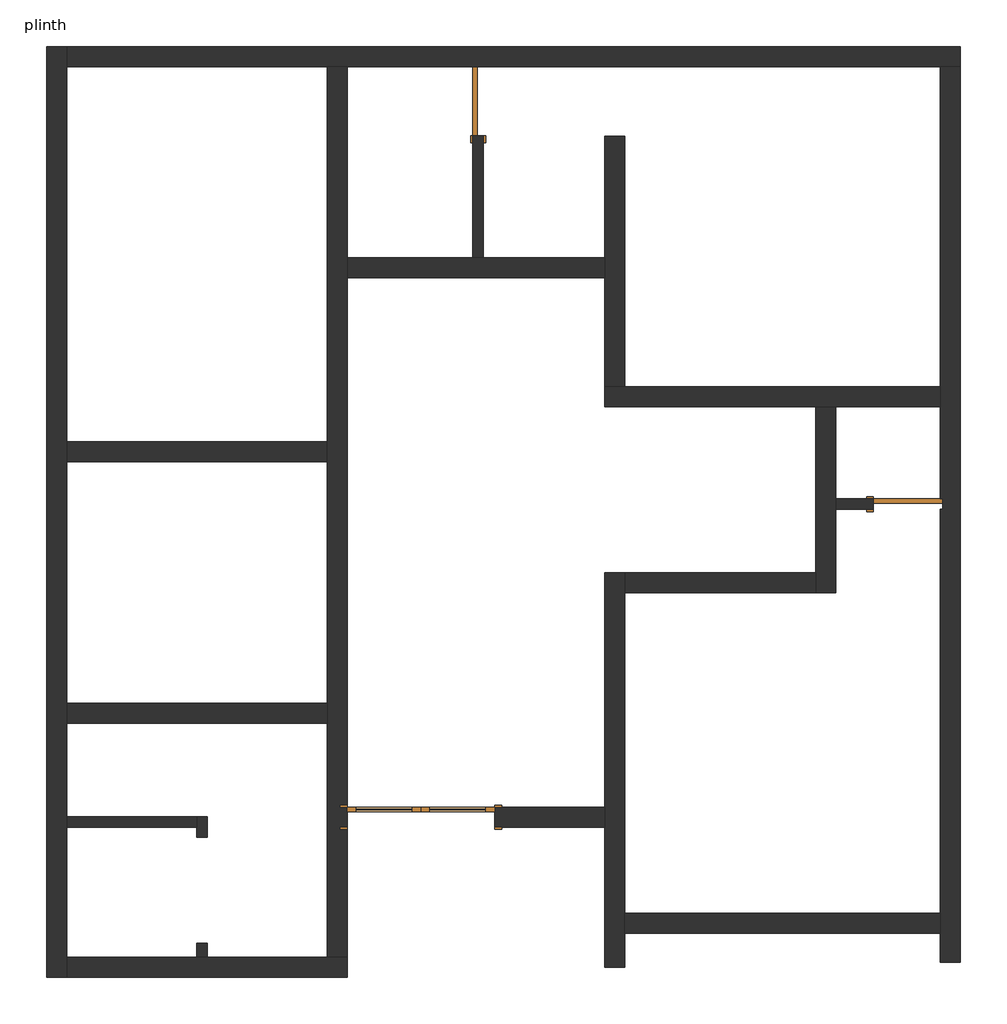
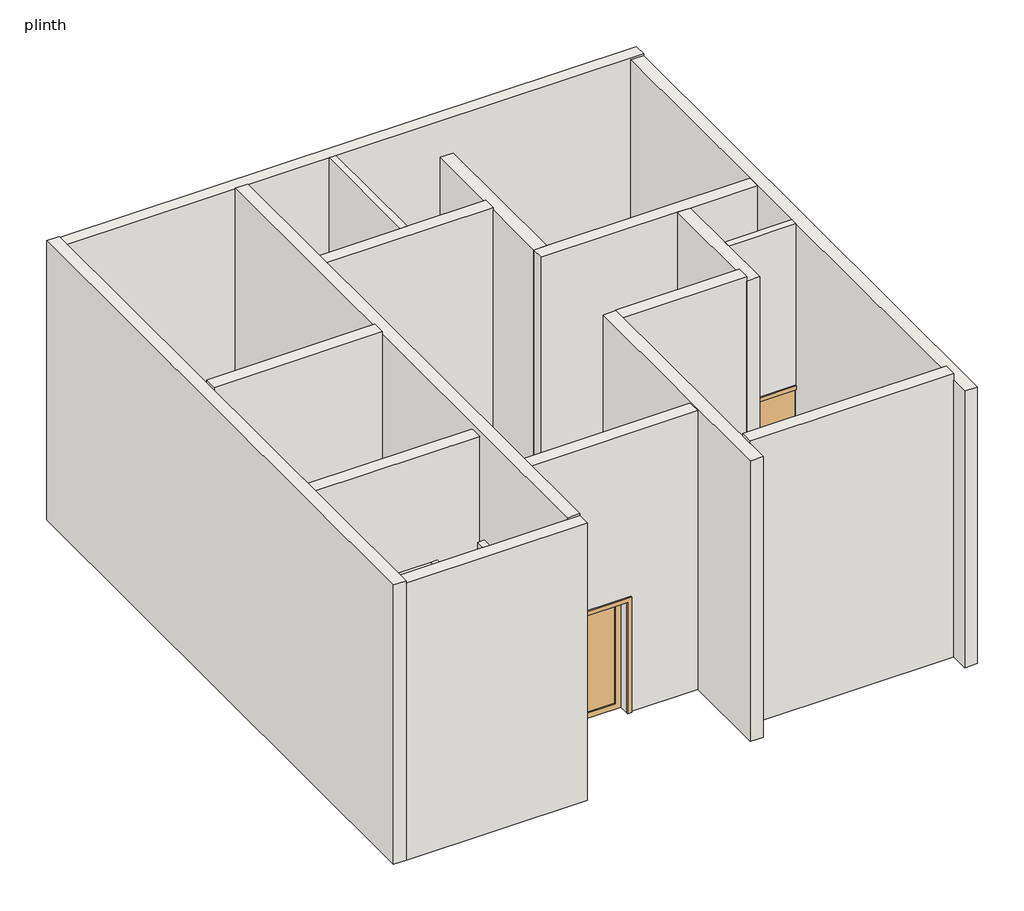
# One storey: 20 walls, 3 doors.
"""IFC4 building model written with IfcOpenShell, lengths in millimetres."""

import ifcopenshell
import ifcopenshell.guid

model = None  # the IFC model being written
_history = None  # IfcOwnerHistory: only IFC2X3 demands one
_inside = {}  # id of a spatial element -> (the spatial element, [elements in it])
_under = {}  # id of a project, library or spatial element -> (it, [spatial elements below it])
_declared = {}  # id of a project -> (the project, [libraries it declares])
_typed = {}  # id of a type object -> (the type object, [elements of that type])
_made_of = {}  # id of a material, layer set ... -> (it, [elements and type objects made of it])


def new_model(schema):
    """Start an empty IFC model of exactly this schema.

    Asked for "IFC4X3", IfcOpenShell would pick the latest addendum, in which some entities
    have other attributes; the version numbers below select the first issue.
    IFC2X3 requires an IfcOwnerHistory on every rooted entity: one is made here for all.
    """
    global model, _history
    if schema == "IFC4X3":
        model = ifcopenshell.file(schema_version=(4, 3, 0, 0))
    else:
        model = ifcopenshell.file(schema=schema)
    _inside.clear()
    _under.clear()
    _declared.clear()
    _typed.clear()
    _made_of.clear()
    _history = None
    if model.schema == "IFC2X3":
        org = make("IfcOrganization", Name="unknown")
        user = make(
            "IfcPersonAndOrganization",
            ThePerson=make("IfcPerson", FamilyName="unknown"),
            TheOrganization=org,
        )
        app = make(
            "IfcApplication",
            ApplicationDeveloper=org,
            Version="unknown",
            ApplicationFullName="unknown",
            ApplicationIdentifier="unknown",
        )
        _history = make(
            "IfcOwnerHistory",
            OwningUser=user,
            OwningApplication=app,
            ChangeAction="ADDED",
            CreationDate=0,
        )
    return model


def make(cls, **values):
    """One entity of the class cls with the attributes given. An attribute that is None is left unset."""
    return model.create_entity(
        cls, **{name: value for name, value in values.items() if value is not None}
    )


def rooted(cls, **values):
    """An entity with a GlobalId (a new one), such as an element, a storey or a relation."""
    return make(cls, GlobalId=ifcopenshell.guid.new(), OwnerHistory=_history, **values)


def si_unit(unit_type, name, prefix=None):
    """IfcSIUnit, for example si_unit("LENGTHUNIT", "METRE", prefix="MILLI")."""
    return make("IfcSIUnit", UnitType=unit_type, Prefix=prefix, Name=name)


def assignment(units):
    """IfcUnitAssignment: the units of a project."""
    return None if units is None else make("IfcUnitAssignment", Units=units)


def point(xyz):
    """IfcCartesianPoint."""
    return None if xyz is None else make("IfcCartesianPoint", Coordinates=xyz)


def direction(xyz):
    """IfcDirection."""
    return None if xyz is None else make("IfcDirection", DirectionRatios=xyz)


def frame(location, z_axis=None, x_axis=None):
    """IfcAxis2Placement3D, a coordinate frame: its origin and axes. An axis left out is left unset."""
    return make(
        "IfcAxis2Placement3D",
        Location=point(location),
        Axis=direction(z_axis),
        RefDirection=direction(x_axis),
    )


def origin():
    """The frame at (0, 0, 0) with its axes left unset."""
    return frame((0.0, 0.0, 0.0))


def origin_with_axes():
    """The frame at (0, 0, 0) with the z axis (0, 0, 1) and the x axis (1, 0, 0) written out."""
    return frame((0.0, 0.0, 0.0), z_axis=(0.0, 0.0, 1.0), x_axis=(1.0, 0.0, 0.0))


def place(relative_to, where):
    """IfcLocalPlacement: puts the frame where relative to a parent placement (None: the world)."""
    return make(
        "IfcLocalPlacement", PlacementRelTo=relative_to, RelativePlacement=where
    )


def context(
    kind, dimensions, precision=None, world=None, true_north=None, identifier=None
):
    """IfcGeometricRepresentationContext, for example the 3D "Model" context."""
    return make(
        "IfcGeometricRepresentationContext",
        ContextIdentifier=identifier,
        ContextType=kind,
        CoordinateSpaceDimension=dimensions,
        Precision=precision,
        WorldCoordinateSystem=world,
        TrueNorth=true_north,
    )


def project(units=None, contexts=None):
    """IfcProject with its units and contexts."""
    return rooted(
        "IfcProject",
        Name="project",
        RepresentationContexts=contexts,
        UnitsInContext=assignment(units),
    )


def spatial(cls, under=None, at=None, **own):
    """A site, building, storey or space (cls), placed at a placement, below another one or the project."""
    s = rooted(cls, ObjectPlacement=at, **own)
    if under is not None:
        _under.setdefault(under.id(), (under, []))[1].append(s)
    return s


def polyline(points):
    """IfcPolyline through the points."""
    return make("IfcPolyline", Points=[point(p) for p in points])


def outline(outer, holes=None, kind="AREA"):
    """IfcArbitraryClosedProfileDef: a profile drawn as a closed curve; with holes, ...WithVoids."""
    if holes is None:
        return make("IfcArbitraryClosedProfileDef", ProfileType=kind, OuterCurve=outer)
    return make(
        "IfcArbitraryProfileDefWithVoids",
        ProfileType=kind,
        OuterCurve=outer,
        InnerCurves=holes,
    )


def extrude(swept, where, along, depth):
    """IfcExtrudedAreaSolid: the profile swept, set in the frame where, extruded along a direction by depth."""
    return make(
        "IfcExtrudedAreaSolid",
        SweptArea=swept,
        Position=where,
        ExtrudedDirection=direction(along),
        Depth=depth,
    )


def faces_of(points, faces, orient=None, outer=None):
    """IfcFace entities. A face is a list of loops; a loop is a list of indices into points, from 0.

    orient and outer hold one flag for each loop. By default every Orientation is true, the
    first loop of a face is its IfcFaceOuterBound and the others are IfcFaceBound.
    """
    made = []
    for i, loops in enumerate(faces):
        bounds = []
        for j, loop in enumerate(loops):
            is_outer = j == 0 if outer is None else outer[i][j]
            bounds.append(
                make(
                    "IfcFaceOuterBound" if is_outer else "IfcFaceBound",
                    Bound=make("IfcPolyLoop", Polygon=[points[k] for k in loop]),
                    Orientation=True if orient is None else orient[i][j],
                )
            )
        made.append(make("IfcFace", Bounds=bounds))
    return made


def faceted_brep(points, faces, orient=None, outer=None, voids=None):
    """IfcFacetedBrep: a solid bounded by flat faces; with voids (closed shells), ...WithVoids."""
    shared = [point(p) for p in points]
    hull = make("IfcClosedShell", CfsFaces=faces_of(shared, faces, orient, outer))
    if voids is None:
        return make("IfcFacetedBrep", Outer=hull)
    return make(
        "IfcFacetedBrepWithVoids",
        Outer=hull,
        Voids=[
            make(cls, CfsFaces=faces_of(shared, fs, o, b)) for cls, fs, o, b in voids
        ],
    )


def shape(context_of_items, identifier, shape_type, items):
    """IfcShapeRepresentation: the items that make up one representation, for example the "Body"."""
    return make(
        "IfcShapeRepresentation",
        ContextOfItems=context_of_items,
        RepresentationIdentifier=identifier,
        RepresentationType=shape_type,
        Items=items,
    )


def source(mapping_origin, context_of_items, identifier, shape_type, items):
    """IfcRepresentationMap: a shape defined once, which mapped items show again and again."""
    return make(
        "IfcRepresentationMap",
        MappingOrigin=mapping_origin,
        MappedRepresentation=shape(context_of_items, identifier, shape_type, items),
    )


def transform(
    local_origin,
    x_axis=None,
    y_axis=None,
    z_axis=None,
    scale=None,
    scale2=None,
    scale3=None,
    uniform=True,
):
    """IfcCartesianTransformationOperator3D, or its non-uniform kind. x_axis, y_axis, z_axis: its Axis1, 2, 3."""
    if uniform:
        return make(
            "IfcCartesianTransformationOperator3D",
            Axis1=direction(x_axis),
            Axis2=direction(y_axis),
            LocalOrigin=point(local_origin),
            Scale=scale,
            Axis3=direction(z_axis),
        )
    return make(
        "IfcCartesianTransformationOperator3DnonUniform",
        Axis1=direction(x_axis),
        Axis2=direction(y_axis),
        LocalOrigin=point(local_origin),
        Scale=scale,
        Axis3=direction(z_axis),
        Scale2=scale2,
        Scale3=scale3,
    )


def mapped(mapping_source, mapping_target):
    """IfcMappedItem: shows the shape of a source again, moved by a transform."""
    return make(
        "IfcMappedItem", MappingSource=mapping_source, MappingTarget=mapping_target
    )


def made_of(thing, what):
    """Note that an element or type object is made of a material, layer set ...; save() writes the relation."""
    if what is not None:
        _made_of.setdefault(what.id(), (what, []))[1].append(thing)
    return thing


def element(
    cls,
    number,
    at=None,
    inside=None,
    cuts=None,
    type_object=None,
    material=None,
    context=None,
    identifier="Body",
    shape_type=None,
    held_by="IfcProductDefinitionShape",
    body=None,
    shapes=None,
    **own,
):
    """One element of the class cls, such as IfcWall. Its Tag is "e" and its number.

    at: its placement. inside: the storey or other place that contains it. cuts: it is an
    opening in that element (IfcRelVoidsElement). A single representation is given by context,
    identifier, shape_type and body (its items); several are given by shapes. held_by: the class
    of the entity that holds the representations. save() writes the other relations.
    """
    e = rooted(cls, Tag="e%d" % number, ObjectPlacement=at, **own)
    if body is not None:
        shapes = [shape(context, identifier, shape_type, body)]
    if shapes is not None:
        e.Representation = make(held_by, Representations=shapes)
    if inside is not None:
        _inside.setdefault(inside.id(), (inside, []))[1].append(e)
    if cuts is not None:
        rooted(
            "IfcRelVoidsElement", RelatingBuildingElement=cuts, RelatedOpeningElement=e
        )
    if type_object is not None:
        _typed.setdefault(type_object.id(), (type_object, []))[1].append(e)
    return made_of(e, material)


def aggregate(whole, parts):
    """IfcRelAggregates: a whole, such as a stair, and the parts it consists of."""
    return rooted("IfcRelAggregates", RelatingObject=whole, RelatedObjects=parts)


def save(model, path):
    """Write the relations noted so far, then the file.

    IfcRelAggregates (storeys below a building ...), IfcRelContainedInSpatialStructure (elements
    in a storey), IfcRelDefinesByType, IfcRelAssociatesMaterial and IfcRelDeclares: one each for
    every whole, place, type object, material and project.
    """
    for whole, parts in _under.values():
        aggregate(whole, parts)
    for where, things in _inside.values():
        rooted(
            "IfcRelContainedInSpatialStructure",
            RelatedElements=things,
            RelatingStructure=where,
        )
    for kind, things in _typed.values():
        rooted("IfcRelDefinesByType", RelatedObjects=things, RelatingType=kind)
    for what, things in _made_of.values():
        rooted("IfcRelAssociatesMaterial", RelatedObjects=things, RelatingMaterial=what)
    for by, libraries in _declared.values():
        rooted("IfcRelDeclares", RelatingContext=by, RelatedDefinitions=libraries)
    model.write(path)


def m_door_double_glass_1700_x_2100mm_d150df18(model_context):
    return source(origin(), model_context, "Body", "SweptSolid", [
        extrude(outline(polyline([(2100.0, -850.0), (0.0, -850.0), (0.0, 0.0), (2100.0, 0.0), (2100.0, -850.0)]), holes=[polyline([(2000.0, -750.0), (2000.0, -100.0), (100.0, -100.0), (100.0, -750.0), (2000.0, -750.0)])]), frame((0.0, 67.38125, 0.0), z_axis=(0.0, 1.0, 0.0), x_axis=(0.0, 0.0, 1.0)), (0.0, 0.0, 1.0), 50.0),
        extrude(outline(polyline([(2100.0, 850.0), (2100.0, 0.0), (0.0, 0.0), (0.0, 850.0), (2100.0, 850.0)]), holes=[polyline([(2000.0, 750.0), (100.0, 750.0), (100.0, 100.0), (2000.0, 100.0), (2000.0, 750.0)])]), frame((0.0, 67.38125, 0.0), z_axis=(0.0, 1.0, 0.0), x_axis=(0.0, 0.0, 1.0)), (0.0, 0.0, 1.0), 50.0),
        extrude(outline(polyline([(100.0, 95.55625), (750.0, 95.55625), (750.0, 89.20625), (100.0, 89.20625), (100.0, 95.55625)])), frame((0.0, 0.0, 100.0), z_axis=(0.0, 0.0, 1.0), x_axis=(1.0, 0.0, 0.0)), (0.0, 0.0, 1.0), 1900.0),
        extrude(outline(polyline([(-750.0, 95.55625), (-100.0, 95.55625), (-100.0, 89.20625), (-750.0, 89.20625), (-750.0, 95.55625)])), frame((0.0, 0.0, 100.0), z_axis=(0.0, 0.0, 1.0), x_axis=(1.0, 0.0, 0.0)), (0.0, 0.0, 1.0), 1900.0),
        extrude(outline(polyline([(0.0, 930.0), (2180.0, 930.0), (2180.0, -930.0), (0.0, -930.0), (0.0, -850.0), (2100.0, -850.0), (2100.0, 850.0), (0.0, 850.0), (0.0, 930.0)])), frame((0.0, 117.38125, 0.0), z_axis=(0.0, 1.0, 0.0), x_axis=(0.0, 0.0, 1.0)), (0.0, 0.0, 1.0), 25.0),
        extrude(outline(polyline([(0.0, 930.0), (2180.0, 930.0), (2180.0, -930.0), (0.0, -930.0), (0.0, -850.0), (2100.0, -850.0), (2100.0, 850.0), (0.0, 850.0), (0.0, 930.0)])), frame((0.0, -137.61875, 0.0), z_axis=(0.0, 1.0, 0.0), x_axis=(0.0, 0.0, 1.0)), (0.0, 0.0, 1.0), 25.0),
    ])


def m_door_single_panel_800_x_2100mm_7e59a417(model_context):
    return source(origin(), model_context, "Body", "SweptSolid", [
        extrude(outline(polyline([(400.0, 10.0), (-400.0, 10.0), (-400.0, 60.0), (400.0, 60.0), (400.0, 10.0)])), origin_with_axes(), (0.0, 0.0, 1.0), 2100.0),
        extrude(outline(polyline([(2176.2, -476.2), (0.0, -476.2), (0.0, -400.0), (2100.0, -400.0), (2100.0, 400.0), (0.0, 400.0), (0.0, 476.2), (2176.2, 476.2), (2176.2, -476.2)])), frame((0.0, 60.0, 0.0), z_axis=(0.0, 1.0, 0.0), x_axis=(0.0, 0.0, 1.0)), (0.0, 0.0, 1.0), 25.0),
        extrude(outline(polyline([(2176.2, 476.2), (2176.2, -476.2), (0.0, -476.2), (0.0, -400.0), (2100.0, -400.0), (2100.0, 400.0), (0.0, 400.0), (0.0, 476.2), (2176.2, 476.2)])), frame((0.0, -85.0, 0.0), z_axis=(0.0, 1.0, 0.0), x_axis=(0.0, 0.0, 1.0)), (0.0, 0.0, 1.0), 25.0),
    ])


model = new_model("IFC4")

# Units and contexts
model_context = context("Model", 3, world=origin())
ifc_project = project(units=[si_unit("LENGTHUNIT", "METRE", prefix="MILLI")], contexts=[model_context])

# Site, building, storey
site = spatial("IfcSite", under=ifc_project)
building = spatial("IfcBuilding", under=site)
storey = spatial("IfcBuildingStorey", under=building, Name="plinth", Elevation=450.0)

# Doors
placement = place(None, origin())
m_door_double_glass_1700_x_2100mm_shape = m_door_double_glass_1700_x_2100mm_d150df18(model_context)
element("IfcDoor", 1, ObjectType="M_Door-Double-Glass : 1700 x 2100mm", at=placement, inside=storey, context=model_context, shape_type="MappedRepresentation", body=[
    mapped(m_door_double_glass_1700_x_2100mm_shape, transform((-60244.5979307, 16200.8803218, 450.0), x_axis=(1.0, 0.0, 0.0), y_axis=(0.0, 1.0, 0.0), z_axis=(0.0, 0.0, 1.0))),
])
m_door_single_panel_800_x_2100mm_shape = m_door_single_panel_800_x_2100mm_7e59a417(model_context)
element("IfcDoor", 2, ObjectType="M_Door-Single-Panel : 800 x 2100mm", at=placement, inside=storey, context=model_context, shape_type="MappedRepresentation", body=[
    mapped(m_door_single_panel_800_x_2100mm_shape, transform((-54634.742358, 19808.2615718, 450.0), x_axis=(1.0, 0.0, 0.0), y_axis=(0.0, 1.0, 0.0), z_axis=(0.0, 0.0, 1.0))),
])
element("IfcDoor", 3, ObjectType="M_Door-Single-Panel : 800 x 2100mm", at=placement, inside=storey, context=model_context, shape_type="MappedRepresentation", body=[
    mapped(m_door_single_panel_800_x_2100mm_shape, transform((-59584.5979307, 24448.2615718, 450.0), x_axis=(0.0, 1.0, 0.0), y_axis=(-1.0, 0.0, 0.0), z_axis=(0.0, 0.0, 1.0))),
])

# Walls
element("IfcWall", 4, ObjectType="11", at=placement, inside=storey, context=model_context, shape_type="SweptSolid", body=[
    extrude(outline(polyline([(22648.2615718, 5703.6205758), (24848.2615718, 5703.6205758), (24848.2615718, 2550.0), (24048.2615718, 2550.0), (24048.2615718, 450.0), (22648.2615718, 450.0), (22648.2615718, 5703.6205758)])), frame((-59644.5979307, 0.0, 0.0), z_axis=(1.0, 0.0, 0.0), x_axis=(0.0, 1.0, 0.0)), (0.0, 0.0, 1.0), 120.0),
])
element("IfcWall", 5, ObjectType="111", at=placement, inside=storey, context=model_context, shape_type="SweptSolid", body=[
    extrude(outline(polyline([(5670.2151187, -54264.5979307), (5670.2151187, -55464.5979307), (450.0, -55464.5979307), (450.0, -55034.742358), (2550.0, -55034.742358), (2550.0, -54264.5979307), (5670.2151187, -54264.5979307)])), frame((0.0, 19748.2615718, 0.0), z_axis=(0.0, 1.0, 0.0), x_axis=(0.0, 0.0, 1.0)), (0.0, 0.0, 1.0), 120.0),
])
element("IfcWall", 6, ObjectType="111", at=placement, inside=storey, context=model_context, shape_type="Brep", body=[
    faceted_brep([(-62824.5979307, 16208.2615718, 450.0), (-62824.5979307, 16088.2615718, 450.0), (-62824.5979307, 15973.2615718, 450.0), (-62824.5979307, 15973.2615718, 4422.8447483), (-62824.5979307, 16088.2615718, 4422.8447483), (-62824.5979307, 16208.2615718, 4422.8447483), (-62704.5979307, 16208.2615718, 450.0), (-62704.5979307, 16208.2615718, 4422.8447483), (-62704.5979307, 15973.2615718, 4422.8447483), (-62704.5979307, 15973.2615718, 450.0)], [[[0, 1, 2, 3, 4, 5]], [[6, 7, 8, 9]], [[2, 1, 0, 6, 9]], [[3, 2, 9, 8]], [[5, 4, 3, 8, 7]], [[0, 5, 7, 6]]]),
])
element("IfcWall", 7, ObjectType="111", at=placement, inside=storey, context=model_context, shape_type="SweptSolid", body=[
    extrude(outline(polyline([(-62704.5979307, 14753.2615718), (-62704.5979307, 14588.2615718), (-62824.5979307, 14588.2615718), (-62824.5979307, 14753.2615718), (-62704.5979307, 14753.2615718)])), frame((0.0, 0.0, 450.0), z_axis=(0.0, 0.0, 1.0), x_axis=(1.0, 0.0, 0.0)), (0.0, 0.0, 1.0), 5233.6602815),
])
element("IfcWall", 8, ObjectType="111", at=placement, inside=storey, context=model_context, shape_type="SweptSolid", body=[
    extrude(outline(polyline([(-64324.5979307, 16208.2615718), (-62824.5979307, 16208.2615718), (-62824.5979307, 16088.2615718), (-64324.5979307, 16088.2615718), (-64324.5979307, 16208.2615718)])), frame((0.0, 0.0, 450.0), z_axis=(0.0, 0.0, 1.0), x_axis=(1.0, 0.0, 0.0)), (0.0, 0.0, 1.0), 3972.8447483),
])
element("IfcWall", 9, ObjectType="Generic - 200mm", at=placement, inside=storey, context=model_context, shape_type="Brep", body=[
    faceted_brep([(-64554.5979307, 25078.2615718, 450.0), (-64554.5979307, 14358.2615718, 450.0), (-64554.5979307, 14358.2615718, 5718.8262298), (-64554.5979307, 25078.2615718, 5718.8262298), (-64324.5979307, 25078.2615718, 450.0), (-64324.5979307, 25078.2615718, 5700.4423551), (-64324.5979307, 25078.2615718, 5718.8262298), (-64324.5979307, 14358.2615718, 5718.8262298), (-64324.5979307, 14358.2615718, 5683.6602815), (-64324.5979307, 14358.2615718, 450.0), (-64324.5979307, 14588.2615718, 450.0), (-64324.5979307, 16088.2615718, 450.0), (-64324.5979307, 16208.2615718, 450.0), (-64324.5979307, 17288.2615718, 450.0), (-64324.5979307, 17518.2615718, 450.0), (-64324.5979307, 20298.2615718, 450.0), (-64324.5979307, 20528.2615718, 450.0), (-64324.5979307, 24848.2615718, 450.0)], [[[0, 1, 2, 3]], [[4, 5, 6, 7, 8, 9, 10, 11, 12, 13, 14, 15, 16, 17]], [[1, 0, 4, 17, 16, 15, 14, 13, 12, 11, 10, 9]], [[3, 2, 7, 6]], [[2, 1, 9, 8, 7]], [[0, 3, 6, 5, 4]]]),
])
element("IfcWall", 10, ObjectType="Generic - 200mm", at=placement, inside=storey, context=model_context, shape_type="Brep", body=[
    faceted_brep([(-64324.5979307, 14358.2615718, 450.0), (-61094.5979307, 14358.2615718, 450.0), (-61094.5979307, 14358.2615718, 5683.6602815), (-64324.5979307, 14358.2615718, 5683.6602815), (-64324.5979307, 14588.2615718, 450.0), (-64324.5979307, 14588.2615718, 5683.6602815), (-62824.5979307, 14588.2615718, 5683.6602815), (-62704.5979307, 14588.2615718, 5683.6602815), (-61094.5979307, 14588.2615718, 5683.6602815), (-61094.5979307, 14588.2615718, 450.0), (-61324.5979307, 14588.2615718, 450.0), (-62704.5979307, 14588.2615718, 450.0), (-62824.5979307, 14588.2615718, 450.0)], [[[0, 1, 2, 3]], [[4, 5, 6, 7, 8, 9, 10, 11, 12]], [[1, 0, 4, 12, 11, 10, 9]], [[3, 2, 8, 7, 6, 5]], [[0, 3, 5, 4]], [[2, 1, 9, 8]]]),
])
element("IfcWall", 11, ObjectType="Generic - 200mm", at=placement, inside=storey, context=model_context, shape_type="Brep", body=[
    faceted_brep([(-61094.5979307, 14588.2615718, 450.0), (-61094.5979307, 22418.2615718, 450.0), (-61094.5979307, 22648.2615718, 450.0), (-61094.5979307, 24848.2615718, 450.0), (-61094.5979307, 24848.2615718, 5716.9832473), (-61094.5979307, 14588.2615718, 5716.9832473), (-61094.5979307, 14588.2615718, 5683.6602815), (-61324.5979307, 14588.2615718, 450.0), (-61324.5979307, 14588.2615718, 5716.9832473), (-61324.5979307, 24848.2615718, 5716.9832473), (-61324.5979307, 24848.2615718, 450.0), (-61324.5979307, 20528.2615718, 450.0), (-61324.5979307, 20433.9365718, 450.0), (-61324.5979307, 20392.5865718, 450.0), (-61324.5979307, 20298.2615718, 450.0), (-61324.5979307, 17518.2615718, 450.0), (-61324.5979307, 17288.2615718, 450.0), (-61244.5979307, 24848.2615718, 450.0)], [[[0, 1, 2, 3, 4, 5, 6]], [[7, 8, 9, 10, 11, 12, 13, 14, 15, 16]], [[3, 2, 1, 0, 7, 16, 15, 14, 13, 12, 11, 10, 17]], [[5, 4, 9, 8]], [[4, 3, 17, 10, 9]], [[0, 6, 5, 8, 7]]]),
])
element("IfcWall", 12, ObjectType="Generic - 200mm", at=placement, inside=storey, context=model_context, shape_type="Brep", body=[
    faceted_brep([(-54034.5979307, 25078.2615718, 450.0), (-64324.5979307, 25078.2615718, 450.0), (-64324.5979307, 25078.2615718, 5700.4423551), (-54034.5979307, 25078.2615718, 5700.4423551), (-54034.5979307, 24848.2615718, 450.0), (-54034.5979307, 24848.2615718, 5670.2151187), (-54034.5979307, 24848.2615718, 5700.4423551), (-64324.5979307, 24848.2615718, 5700.4423551), (-64324.5979307, 24848.2615718, 450.0), (-61324.5979307, 24848.2615718, 450.0), (-61094.5979307, 24848.2615718, 450.0), (-54264.5979307, 24848.2615718, 450.0)], [[[0, 1, 2, 3]], [[4, 5, 6, 7, 8, 9, 10, 11]], [[1, 0, 4, 11, 10, 9, 8]], [[3, 2, 7, 6]], [[2, 1, 8, 7]], [[0, 3, 6, 5, 4]]]),
])
element("IfcWall", 13, ObjectType="Generic - 200mm", at=placement, inside=storey, context=model_context, shape_type="Brep", body=[
    faceted_brep([(-54264.5979307, 21158.2615718, 450.0), (-57894.5979307, 21158.2615718, 450.0), (-58124.5979307, 21158.2615718, 450.0), (-58124.5979307, 21158.2615718, 5670.2151187), (-57894.5979307, 21158.2615718, 5670.2151187), (-54264.5979307, 21158.2615718, 5670.2151187), (-54264.5979307, 20928.2615718, 450.0), (-54264.5979307, 20928.2615718, 5670.2151187), (-55464.5979307, 20928.2615718, 5670.2151187), (-55694.5979307, 20928.2615718, 5670.2151187), (-58124.5979307, 20928.2615718, 5670.2151187), (-58124.5979307, 20928.2615718, 450.0), (-55694.5979307, 20928.2615718, 450.0), (-55464.5979307, 20928.2615718, 450.0)], [[[0, 1, 2, 3, 4, 5]], [[6, 7, 8, 9, 10, 11, 12, 13]], [[2, 1, 0, 6, 13, 12, 11]], [[5, 4, 3, 10, 9, 8, 7]], [[3, 2, 11, 10]], [[0, 5, 7, 6]]]),
])
element("IfcWall", 14, ObjectType="Generic - 200mm", at=placement, inside=storey, context=model_context, shape_type="SweptSolid", body=[
    extrude(outline(polyline([(-57894.5979307, 15098.2615718), (-54264.5979307, 15098.2615718), (-54264.5979307, 14868.2615718), (-57894.5979307, 14868.2615718), (-57894.5979307, 15098.2615718)])), frame((0.0, 0.0, 450.0), z_axis=(0.0, 0.0, 1.0), x_axis=(1.0, 0.0, 0.0)), (0.0, 0.0, 1.0), 5348.3262298),
])
element("IfcWall", 15, ObjectType="Generic - 200mm", at=placement, inside=storey, context=model_context, shape_type="SweptSolid", body=[
    extrude(outline(polyline([(5712.0029208, -58124.5979307), (5712.0029208, -61094.5979307), (2550.0, -61094.5979307), (2550.0, -59394.5979307), (450.0, -59394.5979307), (450.0, -58124.5979307), (5712.0029208, -58124.5979307)])), frame((0.0, 16088.2615718, 0.0), z_axis=(0.0, 1.0, 0.0), x_axis=(0.0, 0.0, 1.0)), (0.0, 0.0, 1.0), 230.0),
])
element("IfcWall", 16, ObjectType="Generic - 200mm", at=placement, inside=storey, context=model_context, shape_type="SweptSolid", body=[
    extrude(outline(polyline([(-64324.5979307, 17518.2615718), (-61324.5979307, 17518.2615718), (-61324.5979307, 17288.2615718), (-64324.5979307, 17288.2615718), (-64324.5979307, 17518.2615718)])), frame((0.0, 0.0, 450.0), z_axis=(0.0, 0.0, 1.0), x_axis=(1.0, 0.0, 0.0)), (0.0, 0.0, 1.0), 5168.3751777),
])
element("IfcWall", 17, ObjectType="Generic - 200mm", at=placement, inside=storey, context=model_context, shape_type="SweptSolid", body=[
    extrude(outline(polyline([(-64324.5979307, 20528.2615718), (-61324.5979307, 20528.2615718), (-61324.5979307, 20298.2615718), (-64324.5979307, 20298.2615718), (-64324.5979307, 20528.2615718)])), frame((0.0, 0.0, 450.0), z_axis=(0.0, 0.0, 1.0), x_axis=(1.0, 0.0, 0.0)), (0.0, 0.0, 1.0), 5319.7733967),
])
element("IfcWall", 18, ObjectType="Generic - 200mm", at=placement, inside=storey, context=model_context, shape_type="Brep", body=[
    faceted_brep([(-58124.5979307, 22648.2615718, 450.0), (-59524.5979307, 22648.2615718, 450.0), (-59644.5979307, 22648.2615718, 450.0), (-61094.5979307, 22648.2615718, 450.0), (-61094.5979307, 22648.2615718, 5703.6205758), (-59644.5979307, 22648.2615718, 5703.6205758), (-59524.5979307, 22648.2615718, 5703.6205758), (-58124.5979307, 22648.2615718, 5703.6205758), (-58124.5979307, 22418.2615718, 450.0), (-58124.5979307, 22418.2615718, 5703.6205758), (-61094.5979307, 22418.2615718, 5703.6205758), (-61094.5979307, 22418.2615718, 450.0)], [[[0, 1, 2, 3, 4, 5, 6, 7]], [[8, 9, 10, 11]], [[3, 2, 1, 0, 8, 11]], [[7, 6, 5, 4, 10, 9]], [[4, 3, 11, 10]], [[0, 7, 9, 8]]]),
])
element("IfcWall", 19, ObjectType="Generic - 200mm", at=placement, inside=storey, context=model_context, shape_type="Brep", body=[
    faceted_brep([(-58124.5979307, 19018.2615718, 450.0), (-58124.5979307, 16318.2615718, 450.0), (-58124.5979307, 16088.2615718, 450.0), (-58124.5979307, 14473.2615718, 450.0), (-58124.5979307, 14473.2615718, 5742.9767558), (-58124.5979307, 19018.2615718, 5742.9767558), (-57894.5979307, 19018.2615718, 450.0), (-57894.5979307, 19018.2615718, 5742.9767558), (-57894.5979307, 14473.2615718, 5742.9767558), (-57894.5979307, 14473.2615718, 450.0), (-57894.5979307, 14868.2615718, 450.0), (-57894.5979307, 15098.2615718, 450.0), (-57894.5979307, 18788.2615718, 450.0)], [[[0, 1, 2, 3, 4, 5]], [[6, 7, 8, 9, 10, 11, 12]], [[3, 2, 1, 0, 6, 12, 11, 10, 9]], [[4, 3, 9, 8]], [[5, 4, 8, 7]], [[0, 5, 7, 6]]]),
])
element("IfcWall", 20, ObjectType="Generic - 200mm", at=placement, inside=storey, context=model_context, shape_type="Brep", body=[
    faceted_brep([(-57894.5979307, 21158.2615718, 450.0), (-57894.5979307, 24043.2615718, 450.0), (-57894.5979307, 24043.2615718, 5670.2151187), (-57894.5979307, 21158.2615718, 5670.2151187), (-58124.5979307, 21158.2615718, 450.0), (-58124.5979307, 21158.2615718, 5670.2151187), (-58124.5979307, 24043.2615718, 5670.2151187), (-58124.5979307, 24043.2615718, 450.0), (-58124.5979307, 22648.2615718, 450.0), (-58124.5979307, 22418.2615718, 450.0), (-57988.9229307, 21158.2615718, 450.0), (-58030.2729307, 21158.2615718, 450.0)], [[[0, 1, 2, 3]], [[4, 5, 6, 7, 8, 9]], [[1, 0, 10, 11, 4, 9, 8, 7]], [[2, 1, 7, 6]], [[3, 2, 6, 5]], [[0, 3, 5, 4, 11, 10]]]),
])
element("IfcWall", 21, ObjectType="Generic - 200mm", at=placement, inside=storey, context=model_context, shape_type="Brep", body=[
    faceted_brep([(-55464.5979307, 18788.2615718, 450.0), (-55464.5979307, 19748.2615718, 450.0), (-55464.5979307, 19868.2615718, 450.0), (-55464.5979307, 20928.2615718, 450.0), (-55464.5979307, 20928.2615718, 5670.2151187), (-55464.5979307, 19868.2615718, 5670.2151187), (-55464.5979307, 19748.2615718, 5670.2151187), (-55464.5979307, 18788.2615718, 5670.2151187), (-55694.5979307, 18788.2615718, 450.0), (-55694.5979307, 18788.2615718, 5670.2151187), (-55694.5979307, 20928.2615718, 5670.2151187), (-55694.5979307, 20928.2615718, 450.0), (-55694.5979307, 19018.2615718, 450.0)], [[[0, 1, 2, 3, 4, 5, 6, 7]], [[8, 9, 10, 11, 12]], [[3, 2, 1, 0, 8, 12, 11]], [[7, 6, 5, 4, 10, 9]], [[4, 3, 11, 10]], [[0, 7, 9, 8]]]),
])
element("IfcWall", 22, ObjectType="Generic - 200mm", at=placement, inside=storey, context=model_context, shape_type="Brep", body=[
    faceted_brep([(-57894.5979307, 18788.2615718, 450.0), (-55694.5979307, 18788.2615718, 450.0), (-55694.5979307, 18788.2615718, 5670.2151187), (-55694.5979307, 18788.2615718, 5754.54105), (-57894.5979307, 18788.2615718, 5754.54105), (-57894.5979307, 19018.2615718, 450.0), (-57894.5979307, 19018.2615718, 5742.9767558), (-57894.5979307, 19018.2615718, 5754.54105), (-55694.5979307, 19018.2615718, 5754.54105), (-55694.5979307, 19018.2615718, 450.0), (-57894.5979307, 18882.5865718, 450.0), (-57894.5979307, 18923.9365718, 450.0)], [[[0, 1, 2, 3, 4]], [[5, 6, 7, 8, 9]], [[1, 0, 10, 11, 5, 9]], [[4, 3, 8, 7]], [[0, 4, 7, 6, 5, 11, 10]], [[3, 2, 1, 9, 8]]]),
])
element("IfcWall", 23, ObjectType="Generic - 200mm", at=placement, inside=storey, context=model_context, shape_type="Brep", body=[
    faceted_brep([(-54264.5979307, 14533.2615718, 450.0), (-54264.5979307, 14533.2615718, 5670.2151187), (-54264.5979307, 19748.2615718, 5670.2151187), (-54264.5979307, 19868.2615718, 5670.2151187), (-54264.5979307, 20928.2615718, 5670.2151187), (-54264.5979307, 21158.2615718, 5670.2151187), (-54264.5979307, 24848.2615718, 5670.2151187), (-54264.5979307, 24848.2615718, 450.0), (-54264.5979307, 21158.2615718, 450.0), (-54264.5979307, 20928.2615718, 450.0), (-54264.5979307, 19868.2615718, 450.0), (-54264.5979307, 19868.2615718, 2550.0), (-54264.5979307, 19748.2615718, 2550.0), (-54264.5979307, 19748.2615718, 450.0), (-54264.5979307, 15098.2615718, 450.0), (-54264.5979307, 14868.2615718, 450.0), (-54034.5979307, 14533.2615718, 450.0), (-54034.5979307, 24848.2615718, 450.0), (-54034.5979307, 24848.2615718, 5670.2151187), (-54034.5979307, 14533.2615718, 5670.2151187), (-54234.742358, 19748.2615718, 450.0), (-54234.742358, 19868.2615718, 450.0), (-54234.742358, 19748.2615718, 2550.0), (-54234.742358, 19868.2615718, 2550.0)], [[[0, 1, 2, 3, 4, 5, 6, 7, 8, 9, 10, 11, 12, 13, 14, 15]], [[16, 17, 18, 19]], [[17, 16, 0, 15, 14, 13, 20, 21, 10, 9, 8, 7]], [[1, 0, 16, 19]], [[6, 5, 4, 3, 2, 1, 19, 18]], [[7, 6, 18, 17]], [[22, 20, 13, 12]], [[21, 23, 11, 10]], [[20, 22, 23, 21]], [[23, 22, 12, 11]]]),
])

save(model, "model.ifc")

# Revit data of these elements
# Project information
#   Project Issue Date = "Issue Date"
#   Project Status = "Project Status"
#   Client Name = "Owner"
#   Project Address = "Enter address here"
#   Project Name = "Project Name"
#   Project Number = "0001"
# Type "M_Door-Double-Glass : 1700 x 2100mm"
#   Type Mark = "42"
#   Construction Type Id = "opn-d45"
#   Assembly Code = "C1020"
#   Analytic Construction = "Wood frame, double glass door "
#   W = 85 cm
#   Thickness = 5 cm
#   Thermal Resistance (R) = 0.31964 (m²·K)/W
#   Swing Angle [instance default] = 90.00°
#   Heat Transfer Coefficient (U) = 3.12872 W/(m²·K)
#   Height = 210 cm
#   Bottom Rail = 10 cm
#   Top Rail = 10 cm
#   Stiles = 10 cm
#   Trim Projection = 2.5 cm
#   Trim Width = 8 cm
#   Width = 170 cm
#   Glazing = Glass
#   Panel Material = Wood - Birch - Solid Stained Light Low Gloss
#   Trim Material = Paint - Sienna
#   Visual Light Transmittance = 0
#   Solar Heat Gain Coefficient = 0
#   Function = (empty or 0)
#   Wall Closure = (empty or 0)
# Type "M_Door-Single-Panel : 800 x 2100mm"
#   Type Mark = "41"
#   Construction Type Id = "DOOR"
#   Assembly Code = "C1020300"
#   Analytic Construction = "Wooden"
#   Thickness = 5 cm
#   Thermal Resistance (R) = 0.455703 (m²·K)/W
#   Swing Angle [instance default] = 90.00°
#   Heat Transfer Coefficient (U) = 2.19465 W/(m²·K)
#   Height = 210 cm
#   Trim Projection Ext = 2.5 cm
#   Trim Projection Int = 2.5 cm
#   Trim Width = 8 cm
#   Width = 80 cm
#   Panel Material = Wood - Birch - Solid Stained Light Low Gloss
#   Trim Material = Paint - Sienna
#   Visual Light Transmittance = 0
#   Solar Heat Gain Coefficient = 0
#   Function = (empty or 0)
#   Wall Closure = (empty or 0)
# Type "11"
#   Layers, outside or top first: 1 cm no material (function 1); 10 cm no material (function 1); 1 cm no material (function 1)
# Type "111"
#   Layers, outside or top first: 1 cm no material (function 1); 10 cm no material (function 1); 1 cm no material (function 1)
# Type "Generic - 200mm"
#   Layers, outside or top first: 1.5 cm no material (function 1); 20 cm no material (function 1); 1.5 cm no material (function 1)
# Element 1 (IfcDoor, "M_Door-Double-Glass : 1700 x 2100mm")
#   Swing Angle = 90.00°
#   Phase Created = New Construction
#   Materials on its faces: "Wood - Birch - Solid Stained Light Low Gloss", "Paint - Sienna", "Glass"
# Elements 2, 3 (IfcDoor, "M_Door-Single-Panel : 800 x 2100mm")
#   Swing Angle = 90.00°
#   Phase Created = New Construction
#   Materials on its faces: "Paint - Sienna", "Wood - Birch - Solid Stained Light Low Gloss"
# Element 4 (IfcWall, "11")
#   Top Offset = 0 cm
#   Base Offset = 0 cm
#   Unconnected Height = 525.3621 cm
#   wall height = 525.3621 cm
#   Phase Created = New Construction
#   Base Constraint = plinth
#   Materials on its faces: "Default Wall"
# Element 5 (IfcWall, "111")
#   Top Offset = 0 cm
#   Base Offset = 0 cm
#   Unconnected Height = 522.0215 cm
#   wall height = 522.0215 cm
#   Phase Created = New Construction
#   Base Constraint = plinth
#   Materials on its faces: "Default Wall"
# Elements 6, 8 (IfcWall, "111")
#   Top Offset = 0 cm
#   Base Offset = 0 cm
#   Unconnected Height = 397.2845 cm
#   wall height = 397.2845 cm
#   Phase Created = New Construction
#   Base Constraint = plinth
#   Materials on its faces: "Default Wall"
# Element 7 (IfcWall, "111")
#   Top Offset = 0 cm
#   Base Offset = 0 cm
#   Unconnected Height = 523.366 cm
#   wall height = 523.366 cm
#   Phase Created = New Construction
#   Base Constraint = plinth
#   Materials on its faces: "Default Wall"
# Element 9 (IfcWall, "Generic - 200mm")
#   Top Offset = 0 cm
#   Base Offset = 0 cm
#   Unconnected Height = 526.8826 cm
#   wall height = 526.8826 cm
#   Phase Created = New Construction
#   Base Constraint = plinth
#   Materials on its faces: "Default Wall"
# Element 10 (IfcWall, "Generic - 200mm")
#   Top Offset = 0 cm
#   Base Offset = 0 cm
#   Unconnected Height = 523.366 cm
#   wall height = 523.366 cm
#   Phase Created = New Construction
#   Base Constraint = plinth
#   Materials on its faces: "Default Wall"
# Element 11 (IfcWall, "Generic - 200mm")
#   Top Offset = 0 cm
#   Base Offset = 0 cm
#   Unconnected Height = 526.6983 cm
#   wall height = 526.6983 cm
#   Phase Created = New Construction
#   Base Constraint = plinth
#   Materials on its faces: "Default Wall"
# Element 12 (IfcWall, "Generic - 200mm")
#   Top Offset = 0 cm
#   Base Offset = 0 cm
#   Unconnected Height = 525.0442 cm
#   wall height = 525.0442 cm
#   Phase Created = New Construction
#   Base Constraint = plinth
#   Materials on its faces: "Default Wall"
# Elements 13, 20, 21 (IfcWall, "Generic - 200mm")
#   Top Offset = 0 cm
#   Base Offset = 0 cm
#   Unconnected Height = 522.0215 cm
#   wall height = 522.0215 cm
#   Phase Created = New Construction
#   Base Constraint = plinth
#   Materials on its faces: "Default Wall"
# Element 14 (IfcWall, "Generic - 200mm")
#   Top Offset = 0 cm
#   Base Offset = 0 cm
#   Unconnected Height = 534.8326 cm
#   wall height = 534.8326 cm
#   Phase Created = New Construction
#   Base Constraint = plinth
#   Materials on its faces: "Default Wall"
# Element 15 (IfcWall, "Generic - 200mm")
#   Top Offset = 0 cm
#   Base Offset = 0 cm
#   Unconnected Height = 526.2003 cm
#   wall height = 526.2003 cm
#   Phase Created = New Construction
#   Base Constraint = plinth
#   Materials on its faces: "Default Wall"
# Element 16 (IfcWall, "Generic - 200mm")
#   Top Offset = 0 cm
#   Base Offset = 0 cm
#   Unconnected Height = 516.8375 cm
#   wall height = 516.8375 cm
#   Phase Created = New Construction
#   Base Constraint = plinth
#   Materials on its faces: "Default Wall"
# Element 17 (IfcWall, "Generic - 200mm")
#   Top Offset = 0 cm
#   Base Offset = 0 cm
#   Unconnected Height = 531.9773 cm
#   wall height = 531.9773 cm
#   Phase Created = New Construction
#   Base Constraint = plinth
#   Materials on its faces: "Default Wall"
# Element 18 (IfcWall, "Generic - 200mm")
#   Top Offset = 0 cm
#   Base Offset = 0 cm
#   Unconnected Height = 525.3621 cm
#   wall height = 525.3621 cm
#   Phase Created = New Construction
#   Base Constraint = plinth
#   Materials on its faces: "Default Wall"
# Element 19 (IfcWall, "Generic - 200mm")
#   Top Offset = 0 cm
#   Base Offset = 0 cm
#   Unconnected Height = 529.2977 cm
#   wall height = 529.2977 cm
#   Phase Created = New Construction
#   Base Constraint = plinth
#   Materials on its faces: "Default Wall"
# Element 22 (IfcWall, "Generic - 200mm")
#   Top Offset = 0 cm
#   Base Offset = 0 cm
#   Unconnected Height = 530.4541 cm
#   wall height = 530.4541 cm
#   Phase Created = New Construction
#   Base Constraint = plinth
#   Materials on its faces: "Default Wall"
# Element 23 (IfcWall, "Generic - 200mm")
#   Top Offset = -87.9785 cm
#   Base Offset = 0 cm
#   wall height = 522.0215 cm
#   Phase Created = New Construction
#   Base Constraint = plinth
#   Top Constraint = 2nd flr
#   Materials on its faces: "Default Wall"
# Materials
#   "Glass": class "Glass", colour RGB 0 128 192, transparency 0.9, Description = "Soda Lime Glass", Cost = 0
#   "Wood - Birch - Solid Stained Light Low Gloss": class "Wood", colour RGB 210 159 95, transparency 0, Cost = 0
#   "Paint - Sienna": class "Miscellaneous", colour RGB 118 70 51, transparency 0, Cost = 0
#   "Default Wall": class "Miscellaneous", colour RGB 128 128 128, transparency 0, Cost = 0
